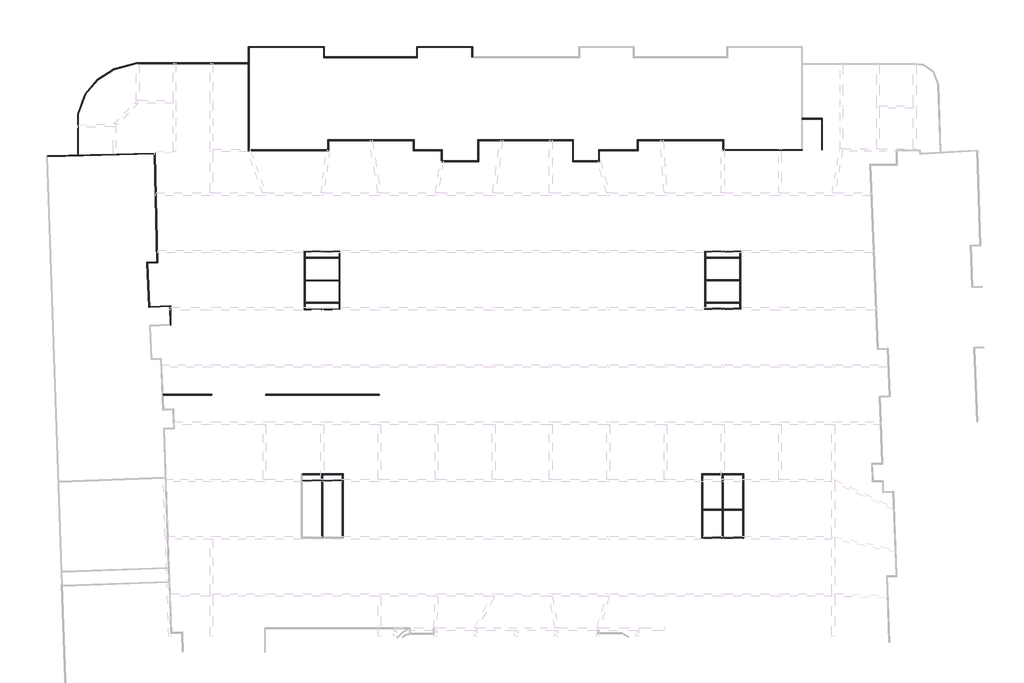
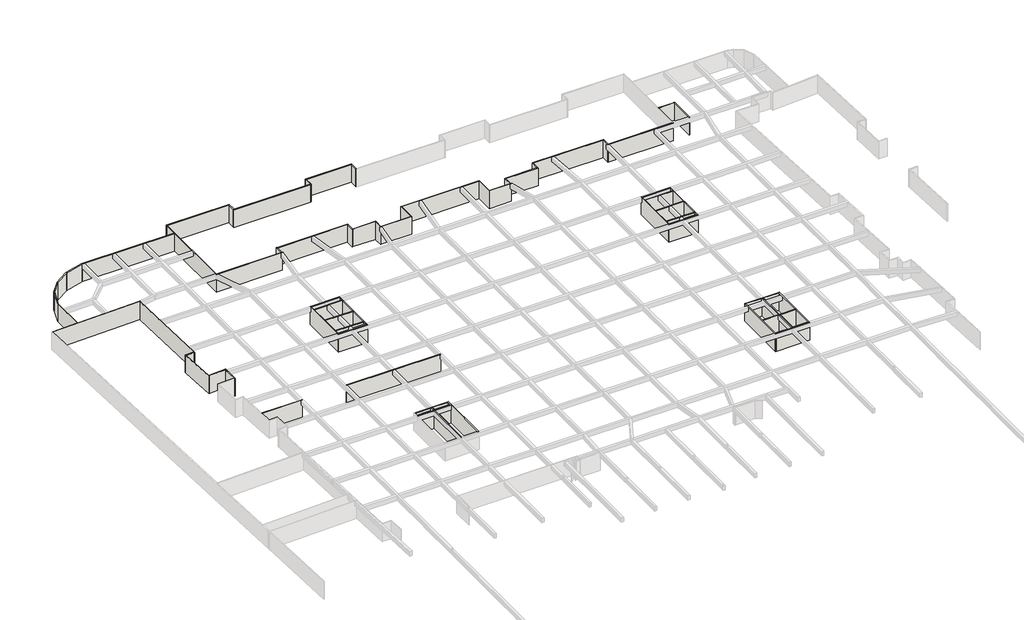
# One storey, part 3 of 8: 64 walls.
# Revit data of these elements (continued)
# Area, not placed, upper offset 0 mm, lower offset 0 mm
#   Number = "64"
#   Name = "fire_compart"
# Area, not placed, upper offset 0 mm, lower offset 0 mm
#   Number = "61"
#   Name = "fire_compart"
# Area, not placed, upper offset 0 mm, lower offset 0 mm
#   Number = "65"
#   Name = "main_building"
# Area, not placed, upper offset 0 mm, lower offset 0 mm
#   Number = "104"
#   Name = "main_building"
# Area, not placed, upper offset 0 mm, lower offset 0 mm
#   Number = "62"
#   Name = "fire_compart"
# Area, not placed, upper offset 0 mm, lower offset 0 mm
#   Number = "125"
#   Name = "fire_compart"
# Area, not placed, upper offset 0 mm, lower offset 0 mm
#   Number = "164"
#   Name = "main_building"
# Area, not placed, upper offset 0 mm, lower offset 0 mm
#   Number = "63"
#   Name = "fire_compart"
# Area, not placed, upper offset 0 mm, lower offset 0 mm
#   Number = "66"
#   Name = "main_building"
# Area, not placed, upper offset 0 mm, lower offset 0 mm
#   Number = "126"
#   Name = "fire_compart"
# Area, not placed, upper offset 0 mm, lower offset 0 mm
#   Number = "83"
#   Name = "fire_compart"
# Area, not placed, upper offset 0 mm, lower offset 0 mm
#   Number = "84"
#   Name = "main_building"
# Area, not placed, upper offset 0 mm, lower offset 0 mm
#   Number = "150"
#   Name = "main_building"
# Area, not placed, upper offset 0 mm, lower offset 0 mm
#   Number = "127"
#   Name = "fire_compart"
# Area, not placed, upper offset 0 mm, lower offset 0 mm
#   Number = "7"
#   Name = "fire_compart_5"
# Area, not placed, upper offset 0 mm, lower offset 0 mm
#   Number = "175"
#   Name = "main_building"
# Area, not placed, upper offset 0 mm, lower offset 0 mm
#   Number = "176"
#   Name = "main_building"
# Area, not placed, upper offset 0 mm, lower offset 0 mm
#   Number = "194"
#   Name = "fire_compart"
# Area, not placed, upper offset 0 mm, lower offset 0 mm
#   Number = "128"
#   Name = "fire_compart"
# Area, not placed, upper offset 0 mm, lower offset 0 mm
#   Number = "162"
#   Name = "main_building"
# Area, not placed, upper offset 0 mm, lower offset 0 mm
#   Number = "129"
#   Name = "fire_compart"
# Area, not placed, upper offset 0 mm, lower offset 0 mm
#   Number = "151"
#   Name = "main_building"
# Area, not placed, upper offset 0 mm, lower offset 0 mm
#   Number = "187"
#   Name = "main_building"
# Area, not placed, upper offset 0 mm, lower offset 0 mm
#   Number = "130"
#   Name = "fire_compart"
# Area, not placed, upper offset 0 mm, lower offset 0 mm
#   Number = "109"
#   Name = "main_building"
# Area, not placed, upper offset 0 mm, lower offset 0 mm
#   Number = "195"
#   Name = "面积"
# Area, not placed, upper offset 0 mm, lower offset 0 mm
#   Number = "196"
#   Name = "fire_compart"
# Area, not placed, upper offset 0 mm, lower offset 0 mm
#   Number = "67"
#   Name = "fire_compart"
# Area, not placed, upper offset 0 mm, lower offset 0 mm
#   Number = "112"
#   Name = "main_building"
# Area, not placed, upper offset 0 mm, lower offset 0 mm
#   Number = "197"
#   Name = "fire_compart"
# Area, not placed, upper offset 0 mm, lower offset 0 mm
#   Number = "198"
#   Name = "fire_compart"
# Area, not placed, upper offset 0 mm, lower offset 0 mm
#   Number = "131"
#   Name = "fire_compart"
# Area, not placed, upper offset 0 mm, lower offset 0 mm
#   Number = "199"
#   Name = "fire_compart"
# Area, not placed, upper offset 0 mm, lower offset 0 mm
#   Number = "68"
#   Name = "fire_compart"
# Area, not placed, upper offset 0 mm, lower offset 0 mm
#   Number = "152"
#   Name = "main_building"
# Area, not placed, upper offset 0 mm, lower offset 0 mm
#   Number = "132"
#   Name = "fire_compart"
# Area, not placed, upper offset 0 mm, lower offset 0 mm
#   Number = "1"
#   Name = "面积"
# Area, not placed, upper offset 0 mm, lower offset 0 mm
#   Number = "2"
#   Name = "防火区域1"
# Area, not placed, upper offset 0 mm, lower offset 0 mm
#   Number = "188"
#   Name = "main_building"
# Area, not placed, upper offset 0 mm, lower offset 0 mm
#   Number = "133"
#   Name = "fire_compart"
# Area, not placed, upper offset 0 mm, lower offset 0 mm
#   Number = "144"
#   Name = "fire_compart"
# Area, not placed, upper offset 0 mm, lower offset 0 mm
#   Number = "200"
#   Name = "fire_compart"
# Area, not placed, upper offset 0 mm, lower offset 0 mm
#   Number = "201"
#   Name = "fire_compart"
# Area, not placed, upper offset 0 mm, lower offset 0 mm
#   Number = "202"
#   Name = "fire_compart"
# Area, not placed, upper offset 0 mm, lower offset 0 mm
#   Number = "134"
#   Name = "fire_compart"
# Area, not placed, upper offset 0 mm, lower offset 0 mm
#   Number = "203"
#   Name = "fire_compart"
# Area, not placed, upper offset 0 mm, lower offset 0 mm
#   Number = "25"
#   Name = "fire_compart"
# Area, not placed, upper offset 0 mm, lower offset 0 mm
#   Number = "26"
#   Name = "fire_compart"
# Area, not placed, upper offset 0 mm, lower offset 0 mm
#   Number = "27"
#   Name = "fire_compart"
# Area, not placed, upper offset 0 mm, lower offset 0 mm
#   Number = "69"
#   Name = "fire_compart"
# Area, not placed, upper offset 0 mm, lower offset 0 mm
#   Number = "105"
#   Name = "main_building"
# Area, not placed, upper offset 0 mm, lower offset 0 mm
#   Number = "113"
#   Name = "main_building"
# Area, not placed, upper offset 0 mm, lower offset 0 mm
#   Number = "153"
#   Name = "main_building"
# Area, not placed, upper offset 0 mm, lower offset 0 mm
#   Number = "177"
#   Name = "main_building"
# Area, not placed, upper offset 0 mm, lower offset 0 mm
#   Number = "135"
#   Name = "fire_compart"
# Area, not placed, upper offset 0 mm, lower offset 0 mm
#   Number = "189"
#   Name = "main_building"
# Area, not placed, upper offset 0 mm, lower offset 0 mm
#   Number = "85"
#   Name = "fire_compart"
# Area, not placed, upper offset 0 mm, lower offset 0 mm
#   Number = "86"
#   Name = "main_building"
# Area, not placed, upper offset 0 mm, lower offset 0 mm
#   Number = "87"
#   Name = "main_building"
# Area, not placed, upper offset 0 mm, lower offset 0 mm
#   Number = "136"
#   Name = "fire_compart"
# Room, not placed, phase "新构造", upper offset 0 mm, lower offset 0 mm
#   Number = "8"
#   Name = "客餐厅"
# Area, not placed, upper offset 0 mm, lower offset 0 mm
#   Number = "70"
#   Name = "main_building"
# Area, not placed, upper offset 0 mm, lower offset 0 mm
#   Number = "156"
#   Name = "fire_compart"
# Area, not placed, upper offset 0 mm, lower offset 0 mm
#   Number = "154"
#   Name = "main_building"
# Area, not placed, upper offset 0 mm, lower offset 0 mm
#   Number = "190"
#   Name = "main_building"
# Area, not placed, upper offset 0 mm, lower offset 0 mm
#   Number = "114"
#   Name = "main_building"
# Area, not placed, upper offset 0 mm, lower offset 0 mm
#   Number = "8"
#   Name = "fire_compart_6"
# Area, not placed, upper offset 0 mm, lower offset 0 mm
#   Number = "137"
#   Name = "fire_compart"
# Area, not placed, upper offset 0 mm, lower offset 0 mm
#   Number = "178"
#   Name = "main_building"
# Area, not placed, upper offset 0 mm, lower offset 0 mm
#   Number = "163"
#   Name = "main_building"
# Area, not placed, upper offset 0 mm, lower offset 0 mm
#   Number = "138"
#   Name = "fire_compart"
# Area, not placed, upper offset 0 mm, lower offset 0 mm
#   Number = "3"
#   Name = "fire_compart_1"
# Area, not placed, upper offset 0 mm, lower offset 0 mm
#   Number = "168"
#   Name = "fire_compart"
# Area at (688121.903, -978535.869) mm, upper offset 0 mm, lower offset 0 mm
#   Number = "213"
#   Name = "fire_compart"
# Area, not placed, upper offset 0 mm, lower offset 0 mm
#   Number = "139"
#   Name = "fire_compart"
# Area, not placed, upper offset 0 mm, lower offset 0 mm
#   Number = "71"
#   Name = "fire_compart"
# Room, not placed, phase "新构造", upper offset 0 mm, lower offset 0 mm
#   Number = "11"
#   Name = "房间"
# Area, not placed, upper offset 0 mm, lower offset 0 mm
#   Number = "140"
#   Name = "fire_compart"
# Area, not placed, upper offset 0 mm, lower offset 0 mm
#   Number = "191"
#   Name = "main_building"
# Area, not placed, upper offset 0 mm, lower offset 0 mm
#   Number = "155"
#   Name = "main_building"
# Area, not placed, upper offset 0 mm, lower offset 0 mm
#   Number = "106"
#   Name = "main_building"
# Room, not placed, phase "新构造", upper offset 0 mm, lower offset 0 mm
#   Number = "12"
#   Name = "房间"
# Area, not placed, upper offset 0 mm, lower offset 0 mm
#   Number = "110"
#   Name = "main_building"
# Area, not placed, upper offset 0 mm, lower offset 0 mm
#   Number = "115"
#   Name = "main_building"
# Area, not placed, upper offset 0 mm, lower offset 0 mm
#   Number = "141"
#   Name = "fire_compart"
# Area, not placed, upper offset 0 mm, lower offset 0 mm
#   Number = "100"
#   Name = "main_building"
# Area, not placed, upper offset 0 mm, lower offset 0 mm
#   Number = "179"
#   Name = "main_building"
# Room, not placed, phase "新构造", upper offset 0 mm, lower offset 0 mm
#   Number = "13"
#   Name = "房间"
# Room, not placed, phase "新构造", upper offset 0 mm, lower offset 0 mm
#   Number = "14"
#   Name = "房间"
# Area, not placed, upper offset 0 mm, lower offset 0 mm
#   Number = "72"
#   Name = "main_building"
# Room, not placed, phase "新构造", upper offset 0 mm, lower offset 0 mm
#   Number = "15"
#   Name = "房间"
# Area, not placed, upper offset 0 mm, lower offset 0 mm
#   Number = "88"
#   Name = "fire_compart"
# Area, not placed, upper offset 0 mm, lower offset 0 mm
#   Number = "192"
#   Name = "main_building"
# Room, not placed, phase "新构造", upper offset 0 mm, lower offset 0 mm
#   Number = "16"
#   Name = "房间"
# Area, not placed, upper offset 0 mm, lower offset 0 mm
#   Number = "28"
#   Name = "面积"
# Area at (714385.213, -913735.455) mm, upper offset 0 mm, lower offset 0 mm
#   Number = "211"
#   Name = "fire_compart"
# Area, not placed, upper offset 0 mm, lower offset 0 mm
#   Number = "73"
#   Name = "fire_compart"
# Area, not placed, upper offset 0 mm, lower offset 0 mm
#   Number = "116"
#   Name = "main_building"
# Area, not placed, upper offset 0 mm, lower offset 0 mm
#   Number = "101"
#   Name = "main_building"
# Area, not placed, upper offset 0 mm, lower offset 0 mm
#   Number = "193"
#   Name = "main_building"
# Room, not placed, phase "新构造", upper offset 0 mm, lower offset 0 mm
#   Number = "17"
#   Name = "房间"
# Area, not placed, upper offset 0 mm, lower offset 0 mm
#   Number = "30"
#   Name = "main_building"
# Area, not placed, upper offset 0 mm, lower offset 0 mm
#   Number = "143"
#   Name = "fire_compart"
# Area, not placed, upper offset 0 mm, lower offset 0 mm
#   Number = "180"
#   Name = "main_building"
# Area at (756752.523, -911614.082) mm, upper offset 0 mm, lower offset 0 mm
#   Number = "212"
#   Name = "fire_compart"
# Area, not placed, upper offset 0 mm, lower offset 0 mm
#   Number = "89"
#   Name = "main_building"
# Area, not placed, upper offset 0 mm, lower offset 0 mm
#   Number = "75"
#   Name = "main_building"
# Area, not placed, upper offset 0 mm, lower offset 0 mm
#   Number = "111"
#   Name = "main_building"
# Area, not placed, upper offset 0 mm, lower offset 0 mm
#   Number = "90"
#   Name = "fire_compart"
# Area, not placed, upper offset 0 mm, lower offset 0 mm
#   Number = "76"
#   Name = "main_building"
# Area, not placed, upper offset 0 mm, lower offset 0 mm
#   Number = "145"
#   Name = "fire_compart"
# Area, not placed, upper offset 0 mm, lower offset 0 mm
#   Number = "146"
#   Name = "fire_compart"
# Area, not placed, upper offset 0 mm, lower offset 0 mm
#   Number = "147"
#   Name = "fire_compart"
# Area at (706044.351, -950482.468) mm, upper offset 0 mm, lower offset 0 mm
#   Number = "214"
#   Name = "fire_compart"
# Area, not placed, upper offset 0 mm, lower offset 0 mm
#   Number = "117"
#   Name = "main_building"
# Area, not placed, upper offset 0 mm, lower offset 0 mm
#   Number = "4"
#   Name = "fire_compart_2"
# Area, not placed, upper offset 0 mm, lower offset 0 mm
#   Number = "77"
#   Name = "main_building"
# Area, not placed, upper offset 0 mm, lower offset 0 mm
#   Number = "181"
#   Name = "main_building"
# Area, not placed, upper offset 0 mm, lower offset 0 mm
#   Number = "159"
#   Name = "fire_compart"
# Area, not placed, upper offset 0 mm, lower offset 0 mm
#   Number = "78"
#   Name = "main_building"
# Area, not placed, upper offset 0 mm, lower offset 0 mm
#   Number = "79"
#   Name = "main_building"
# Area, not placed, upper offset 0 mm, lower offset 0 mm
#   Number = "29"
#   Name = "main_building"
